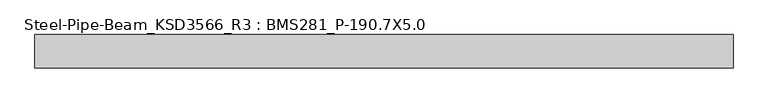
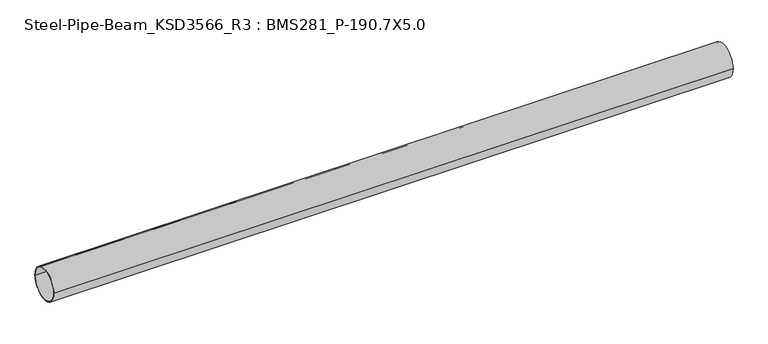
"""IFC4 building model written with IfcOpenShell, lengths in millimetres: member geometry, Steel-Pipe-Beam_KSD3566_R3 : BMS281_P-190.7X5.0."""

from ifc_helpers import new_model, si_unit, point, frame, origin, origin_2d, place, context, project, spatial, circle_curve, trimmed, segment, composite_curve, outline, extrude, source, transform, mapped, element, save


def steel_pipe_beam_ksd3566_r3_bms281_p_190_7x5_0_a2130fa0(model_context):
    return source(origin(), model_context, "Body", "SweptSolid", [
        extrude(outline(composite_curve([segment(trimmed(circle_curve(origin_2d(), 95.35), [point((-95.35, 0.0))], [point((95.35, 0.0))], False, "CARTESIAN"), True, "CONTINUOUS"), segment(trimmed(circle_curve(origin_2d(), 95.35), [point((95.35, 0.0))], [point((-95.35, 0.0))], False, "CARTESIAN"), True, "CONTINUOUS")], self_intersect=False), holes=[composite_curve([segment(trimmed(circle_curve(origin_2d(), 90.35), [point((90.35, 0.0))], [point((-90.35, 0.0))], True, "CARTESIAN"), True, "CONTINUOUS"), segment(trimmed(circle_curve(origin_2d(), 90.35), [point((-90.35, 0.0))], [point((90.35, 0.0))], True, "CARTESIAN"), True, "CONTINUOUS")], self_intersect=False)]), frame((-2046.1374086, 0.0, 0.0), z_axis=(1.0, 0.0, 0.0), x_axis=(0.0, 1.0, 0.0)), (0.0, 0.0, 1.0), 3969.4594784),
    ])


if __name__ == "__main__":
    model = new_model("IFC4")
    model_context = context("Model", 3, world=origin())
    ifc_project = project(units=[si_unit("LENGTHUNIT", "METRE", prefix="MILLI")], contexts=[model_context])
    site = spatial("IfcSite", under=ifc_project)
    building = spatial("IfcBuilding", under=site)
    placement = place(None, origin())
    steel_pipe_beam_ksd3566_r3_bms281_p_190_7x5_0_shape = steel_pipe_beam_ksd3566_r3_bms281_p_190_7x5_0_a2130fa0(model_context)
    element("IfcMember", 1, ObjectType="Steel-Pipe-Beam_KSD3566_R3 : BMS281_P-190.7X5.0", at=placement, inside=building, context=model_context, shape_type="MappedRepresentation", body=[
        mapped(steel_pipe_beam_ksd3566_r3_bms281_p_190_7x5_0_shape, transform((0.0, 0.0, 0.0), x_axis=(1.0, 0.0, 0.0), y_axis=(0.0, 1.0, 0.0), z_axis=(0.0, 0.0, 1.0))),
    ])
    save(model, "model.ifc")

# Revit data of these elements
# Type "Steel-Pipe-Beam_KSD3566_R3 : BMS281_P-190.7X5.0"
#   Keynote = "P-190.7X5.0"
#   SteelWeight = "Light"
#   t = 0.0050 m
#   Surface Area = 0.599102 m²/m
#   Section Area = 29.1697 cm²
#   Mass per Unit Length = 22.8982 kg/m
#   Length [instance default] = 1.5000 m
#   D = 0.1907 m
#   hec_material4 [instance default] = none
#   hec_material3 [instance default] = none
#   hec_material2 [instance default] = none
#   hec_material1 [instance default] = none
#   Structural Material [instance default] = Steel, 45-345
#   Assembly Code = ""
# Element 1 (IfcMember, "Steel-Pipe-Beam_KSD3566_R3 : BMS281_P-190.7X5.0")
#   Structural Material = none
# Materials
#   "Steel, 45-345": class "Metal", colour RGB 189 187 185, transparency 0, Description = "Steel 345 MPa", Cost = 0
